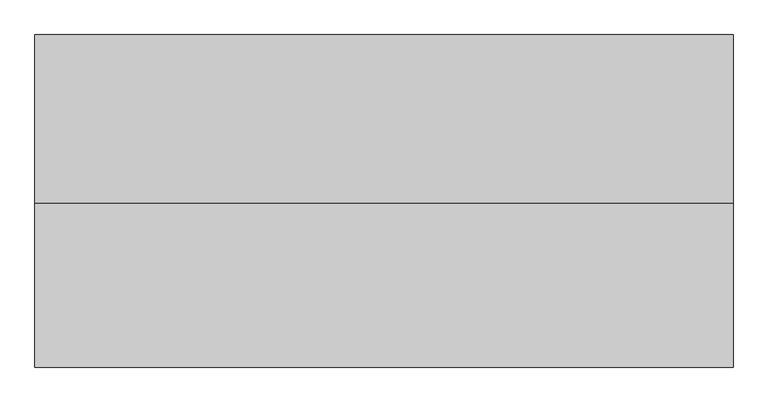
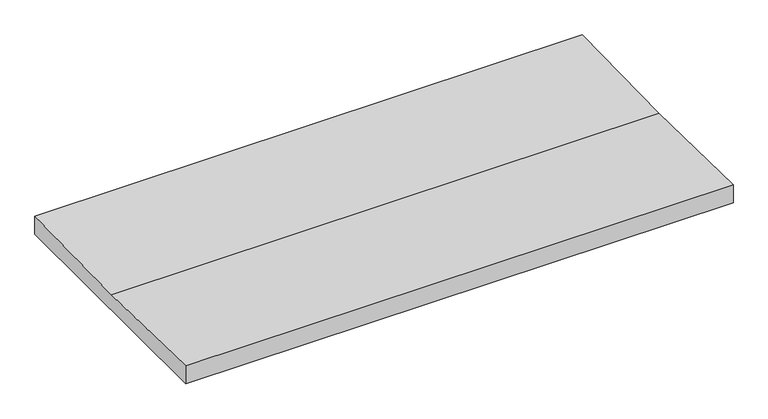
"""IFC4 building model written with IfcOpenShell, lengths in millimetres: proxy geometry, FIRESTONE INSULATION1:FIRESTONE INSULATION001:288590 : FIRESTONE INSULATION1:FIRESTONE INSULATION001:288590."""

import ifcopenshell
import ifcopenshell.guid

model = None  # the IFC model being written
_history = None  # IfcOwnerHistory: only IFC2X3 demands one
_inside = {}  # id of a spatial element -> (the spatial element, [elements in it])
_under = {}  # id of a project, library or spatial element -> (it, [spatial elements below it])
_declared = {}  # id of a project -> (the project, [libraries it declares])
_typed = {}  # id of a type object -> (the type object, [elements of that type])
_made_of = {}  # id of a material, layer set ... -> (it, [elements and type objects made of it])


def new_model(schema):
    """Start an empty IFC model of exactly this schema.

    Asked for "IFC4X3", IfcOpenShell would pick the latest addendum, in which some entities
    have other attributes; the version numbers below select the first issue.
    IFC2X3 requires an IfcOwnerHistory on every rooted entity: one is made here for all.
    """
    global model, _history
    if schema == "IFC4X3":
        model = ifcopenshell.file(schema_version=(4, 3, 0, 0))
    else:
        model = ifcopenshell.file(schema=schema)
    _inside.clear()
    _under.clear()
    _declared.clear()
    _typed.clear()
    _made_of.clear()
    _history = None
    if model.schema == "IFC2X3":
        org = make("IfcOrganization", Name="unknown")
        user = make(
            "IfcPersonAndOrganization",
            ThePerson=make("IfcPerson", FamilyName="unknown"),
            TheOrganization=org,
        )
        app = make(
            "IfcApplication",
            ApplicationDeveloper=org,
            Version="unknown",
            ApplicationFullName="unknown",
            ApplicationIdentifier="unknown",
        )
        _history = make(
            "IfcOwnerHistory",
            OwningUser=user,
            OwningApplication=app,
            ChangeAction="ADDED",
            CreationDate=0,
        )
    return model


def make(cls, **values):
    """One entity of the class cls with the attributes given. An attribute that is None is left unset."""
    return model.create_entity(
        cls, **{name: value for name, value in values.items() if value is not None}
    )


def rooted(cls, **values):
    """An entity with a GlobalId (a new one), such as an element, a storey or a relation."""
    return make(cls, GlobalId=ifcopenshell.guid.new(), OwnerHistory=_history, **values)


def si_unit(unit_type, name, prefix=None):
    """IfcSIUnit, for example si_unit("LENGTHUNIT", "METRE", prefix="MILLI")."""
    return make("IfcSIUnit", UnitType=unit_type, Prefix=prefix, Name=name)


def assignment(units):
    """IfcUnitAssignment: the units of a project."""
    return None if units is None else make("IfcUnitAssignment", Units=units)


def point(xyz):
    """IfcCartesianPoint."""
    return None if xyz is None else make("IfcCartesianPoint", Coordinates=xyz)


def direction(xyz):
    """IfcDirection."""
    return None if xyz is None else make("IfcDirection", DirectionRatios=xyz)


def frame(location, z_axis=None, x_axis=None):
    """IfcAxis2Placement3D, a coordinate frame: its origin and axes. An axis left out is left unset."""
    return make(
        "IfcAxis2Placement3D",
        Location=point(location),
        Axis=direction(z_axis),
        RefDirection=direction(x_axis),
    )


def origin():
    """The frame at (0, 0, 0) with its axes left unset."""
    return frame((0.0, 0.0, 0.0))


def place(relative_to, where):
    """IfcLocalPlacement: puts the frame where relative to a parent placement (None: the world)."""
    return make(
        "IfcLocalPlacement", PlacementRelTo=relative_to, RelativePlacement=where
    )


def context(
    kind, dimensions, precision=None, world=None, true_north=None, identifier=None
):
    """IfcGeometricRepresentationContext, for example the 3D "Model" context."""
    return make(
        "IfcGeometricRepresentationContext",
        ContextIdentifier=identifier,
        ContextType=kind,
        CoordinateSpaceDimension=dimensions,
        Precision=precision,
        WorldCoordinateSystem=world,
        TrueNorth=true_north,
    )


def project(units=None, contexts=None):
    """IfcProject with its units and contexts."""
    return rooted(
        "IfcProject",
        Name="project",
        RepresentationContexts=contexts,
        UnitsInContext=assignment(units),
    )


def spatial(cls, under=None, at=None, **own):
    """A site, building, storey or space (cls), placed at a placement, below another one or the project."""
    s = rooted(cls, ObjectPlacement=at, **own)
    if under is not None:
        _under.setdefault(under.id(), (under, []))[1].append(s)
    return s


def polyline(points):
    """IfcPolyline through the points."""
    return make("IfcPolyline", Points=[point(p) for p in points])


def outline(outer, holes=None, kind="AREA"):
    """IfcArbitraryClosedProfileDef: a profile drawn as a closed curve; with holes, ...WithVoids."""
    if holes is None:
        return make("IfcArbitraryClosedProfileDef", ProfileType=kind, OuterCurve=outer)
    return make(
        "IfcArbitraryProfileDefWithVoids",
        ProfileType=kind,
        OuterCurve=outer,
        InnerCurves=holes,
    )


def extrude(swept, where, along, depth):
    """IfcExtrudedAreaSolid: the profile swept, set in the frame where, extruded along a direction by depth."""
    return make(
        "IfcExtrudedAreaSolid",
        SweptArea=swept,
        Position=where,
        ExtrudedDirection=direction(along),
        Depth=depth,
    )


def shape(context_of_items, identifier, shape_type, items):
    """IfcShapeRepresentation: the items that make up one representation, for example the "Body"."""
    return make(
        "IfcShapeRepresentation",
        ContextOfItems=context_of_items,
        RepresentationIdentifier=identifier,
        RepresentationType=shape_type,
        Items=items,
    )


def source(mapping_origin, context_of_items, identifier, shape_type, items):
    """IfcRepresentationMap: a shape defined once, which mapped items show again and again."""
    return make(
        "IfcRepresentationMap",
        MappingOrigin=mapping_origin,
        MappedRepresentation=shape(context_of_items, identifier, shape_type, items),
    )


def transform(
    local_origin,
    x_axis=None,
    y_axis=None,
    z_axis=None,
    scale=None,
    scale2=None,
    scale3=None,
    uniform=True,
):
    """IfcCartesianTransformationOperator3D, or its non-uniform kind. x_axis, y_axis, z_axis: its Axis1, 2, 3."""
    if uniform:
        return make(
            "IfcCartesianTransformationOperator3D",
            Axis1=direction(x_axis),
            Axis2=direction(y_axis),
            LocalOrigin=point(local_origin),
            Scale=scale,
            Axis3=direction(z_axis),
        )
    return make(
        "IfcCartesianTransformationOperator3DnonUniform",
        Axis1=direction(x_axis),
        Axis2=direction(y_axis),
        LocalOrigin=point(local_origin),
        Scale=scale,
        Axis3=direction(z_axis),
        Scale2=scale2,
        Scale3=scale3,
    )


def mapped(mapping_source, mapping_target):
    """IfcMappedItem: shows the shape of a source again, moved by a transform."""
    return make(
        "IfcMappedItem", MappingSource=mapping_source, MappingTarget=mapping_target
    )


def made_of(thing, what):
    """Note that an element or type object is made of a material, layer set ...; save() writes the relation."""
    if what is not None:
        _made_of.setdefault(what.id(), (what, []))[1].append(thing)
    return thing


def element(
    cls,
    number,
    at=None,
    inside=None,
    cuts=None,
    type_object=None,
    material=None,
    context=None,
    identifier="Body",
    shape_type=None,
    held_by="IfcProductDefinitionShape",
    body=None,
    shapes=None,
    **own,
):
    """One element of the class cls, such as IfcWall. Its Tag is "e" and its number.

    at: its placement. inside: the storey or other place that contains it. cuts: it is an
    opening in that element (IfcRelVoidsElement). A single representation is given by context,
    identifier, shape_type and body (its items); several are given by shapes. held_by: the class
    of the entity that holds the representations. save() writes the other relations.
    """
    e = rooted(cls, Tag="e%d" % number, ObjectPlacement=at, **own)
    if body is not None:
        shapes = [shape(context, identifier, shape_type, body)]
    if shapes is not None:
        e.Representation = make(held_by, Representations=shapes)
    if inside is not None:
        _inside.setdefault(inside.id(), (inside, []))[1].append(e)
    if cuts is not None:
        rooted(
            "IfcRelVoidsElement", RelatingBuildingElement=cuts, RelatedOpeningElement=e
        )
    if type_object is not None:
        _typed.setdefault(type_object.id(), (type_object, []))[1].append(e)
    return made_of(e, material)


def aggregate(whole, parts):
    """IfcRelAggregates: a whole, such as a stair, and the parts it consists of."""
    return rooted("IfcRelAggregates", RelatingObject=whole, RelatedObjects=parts)


def save(model, path):
    """Write the relations noted so far, then the file.

    IfcRelAggregates (storeys below a building ...), IfcRelContainedInSpatialStructure (elements
    in a storey), IfcRelDefinesByType, IfcRelAssociatesMaterial and IfcRelDeclares: one each for
    every whole, place, type object, material and project.
    """
    for whole, parts in _under.values():
        aggregate(whole, parts)
    for where, things in _inside.values():
        rooted(
            "IfcRelContainedInSpatialStructure",
            RelatedElements=things,
            RelatingStructure=where,
        )
    for kind, things in _typed.values():
        rooted("IfcRelDefinesByType", RelatedObjects=things, RelatingType=kind)
    for what, things in _made_of.values():
        rooted("IfcRelAssociatesMaterial", RelatedObjects=things, RelatingMaterial=what)
    for by, libraries in _declared.values():
        rooted("IfcRelDeclares", RelatingContext=by, RelatedDefinitions=libraries)
    model.write(path)


def generic_models_85221339(model_context):
    return source(origin(), model_context, "Body", "SweptSolid", [
        extrude(outline(polyline([(-5064.9256348, 40131.746), (-5064.9256348, 40201.5164062), (-4594.6286758, 40191.7185529), (-4111.9829229, 40201.5164062), (-4111.9829229, 40131.746), (-5064.9256348, 40131.746)])), frame((17159.7769925, 0.0, 0.0), z_axis=(1.0, 0.0, 0.0), x_axis=(0.0, 1.0, 0.0)), (0.0, 0.0, 1.0), 2000.25),
    ])


if __name__ == "__main__":
    model = new_model("IFC4")
    model_context = context("Model", 3, world=origin())
    ifc_project = project(units=[si_unit("LENGTHUNIT", "METRE", prefix="MILLI")], contexts=[model_context])
    site = spatial("IfcSite", under=ifc_project)
    building = spatial("IfcBuilding", under=site)
    placement = place(None, origin())
    generic_models_shape = generic_models_85221339(model_context)
    element("IfcBuildingElementProxy", 1, Name="FIRESTONE INSULATION1:FIRESTONE INSULATION001:288590 : FIRESTONE INSULATION1:FIRESTONE INSULATION001:288590", ObjectType="FIRESTONE INSULATION1:FIRESTONE INSULATION001:288590 : FIRESTONE INSULATION1:FIRESTONE INSULATION001:288590", at=placement, inside=building, context=model_context, shape_type="MappedRepresentation", body=[
        mapped(generic_models_shape, transform((0.0, 0.0, 0.0), x_axis=(1.0, 0.0, 0.0), y_axis=(0.0, 1.0, 0.0), z_axis=(0.0, 0.0, 1.0))),
    ])
    save(model, "model.ifc")

# Revit data of these elements
# Type "FIRESTONE INSULATION1:FIRESTONE INSULATION001:288590 : FIRESTONE INSULATION1:FIRESTONE INSULATION001:288590"
#   NameOverride = "FIRESTONE INSULATION1:FIRESTONE INSULATION001:288590"
#   ObjectTypeOverride = "FIRESTONE INSULATION1:FIRESTONE INSULATION001"
#   Reference = "FIRESTONE INSULATION001"
#   Category = "Generic Models"
#   Tag = "288590"
# Element 1 (IfcBuildingElementProxy, "FIRESTONE INSULATION1:FIRESTONE INSULATION001:288590 : FIRESTONE INSULATION1:FIRESTONE INSULATION001:288590")
#   Materials on its faces: "TAPERED 2X SLEEPERS - SLOPED TO DRAIN"
# Materials
#   "TAPERED 2X SLEEPERS - SLOPED TO DRAIN": class "Unassigned", colour RGB 234 198 178, transparency 0
